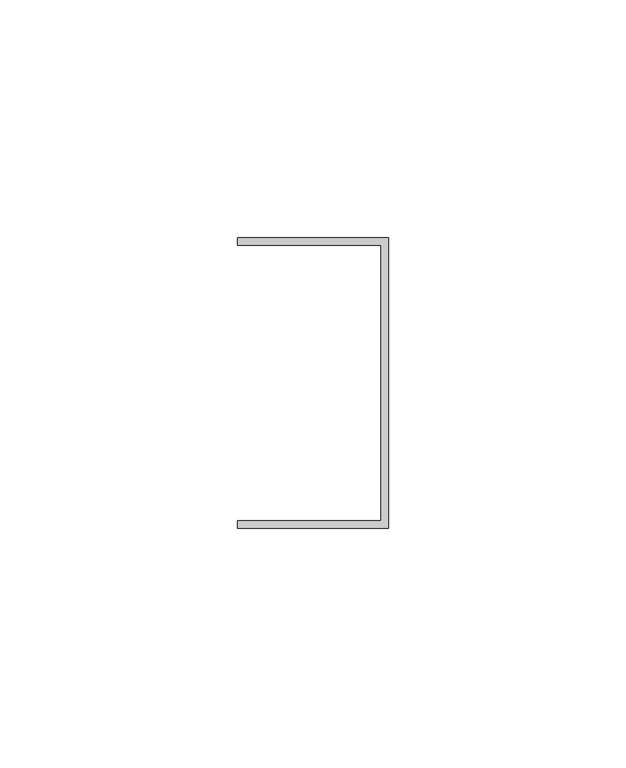
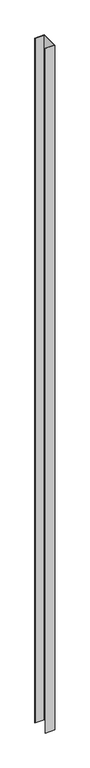
"""IFC4 building model written with IfcOpenShell, lengths in millimetres: proxy geometry, Generic Models 7:Generic Models 1:3:Generic Models 1:3 : Generic Models 7:Generic Models 1:305549:3:Generic Models 1:3:Generic Models 1:3 : Generic Models 7:Generic Models 1:305549:3 : Generic Models 7:Generic Models 1:3:Generic Models 1:3 : Generic Models 7:Generic Models 1:305549:301244:11 : Generic Models 7:Generic Models 1:3:Generic Models 1:3 : Generic Models 7:Generic Models 1:305549:3:Generic Models 1:3:Generic Models 1:3 : Generic Models 7:Generic Models 1:305549:3 : Generic Models 7:Generic Models 1:3:Generic Models 1:3 : Generic Models 7:Generic Models 1:305549:301244:308848."""

from ifc_helpers import new_model, si_unit, frame, origin, place, context, project, spatial, polyline, outline, extrude, source, transform, mapped, element, save


def generic_models_2c4264b5(model_context):
    return source(origin(), model_context, "Body", "SweptSolid", [
        extrude(outline(polyline([(579320.411724, -579015.772634), (579320.411724, -579076.8913841), (579288.661724, -579076.8913841), (579288.661724, -579075.3038841), (579318.824224, -579075.3038841), (579318.824224, -579017.360134), (579288.661724, -579017.360134), (579288.661724, -579015.772634), (579320.411724, -579015.772634)])), frame((0.0, 0.0, 3721.1), z_axis=(0.0, 0.0, 1.0), x_axis=(1.0, 0.0, 0.0)), (0.0, 0.0, 1.0), 2430.9324376),
    ])


if __name__ == "__main__":
    model = new_model("IFC4")
    model_context = context("Model", 3, world=origin())
    ifc_project = project(units=[si_unit("LENGTHUNIT", "METRE", prefix="MILLI")], contexts=[model_context])
    site = spatial("IfcSite", under=ifc_project)
    building = spatial("IfcBuilding", under=site)
    placement = place(None, origin())
    generic_models_shape = generic_models_2c4264b5(model_context)
    element("IfcBuildingElementProxy", 1, Name="Generic Models 7:Generic Models 1:3:Generic Models 1:3 : Generic Models 7:Generic Models 1:305549:3:Generic Models 1:3:Generic Models 1:3 : Generic Models 7:Generic Models 1:305549:3 : Generic Models 7:Generic Models 1:3:Generic Models 1:3 : Generic Models 7:Generic Models 1:305549:301244:11 : Generic Models 7:Generic Models 1:3:Generic Models 1:3 : Generic Models 7:Generic Models 1:305549:3:Generic Models 1:3:Generic Models 1:3 : Generic Models 7:Generic Models 1:305549:3 : Generic Models 7:Generic Models 1:3:Generic Models 1:3 : Generic Models 7:Generic Models 1:305549:301244:308848", ObjectType="Generic Models 7:Generic Models 1:3:Generic Models 1:3 : Generic Models 7:Generic Models 1:305549:3:Generic Models 1:3:Generic Models 1:3 : Generic Models 7:Generic Models 1:305549:3 : Generic Models 7:Generic Models 1:3:Generic Models 1:3 : Generic Models 7:Generic Models 1:305549:301244:11 : Generic Models 7:Generic Models 1:3:Generic Models 1:3 : Generic Models 7:Generic Models 1:305549:3:Generic Models 1:3:Generic Models 1:3 : Generic Models 7:Generic Models 1:305549:3 : Generic Models 7:Generic Models 1:3:Generic Models 1:3 : Generic Models 7:Generic Models 1:305549:301244:308848", at=placement, inside=building, context=model_context, shape_type="MappedRepresentation", body=[
        mapped(generic_models_shape, transform((0.0, 0.0, 0.0), x_axis=(1.0, 0.0, 0.0), y_axis=(0.0, 1.0, 0.0), z_axis=(0.0, 0.0, 1.0))),
    ])
    save(model, "model.ifc")

# Revit data of these elements
# Type "Generic Models 7:Generic Models 1:3:Generic Models 1:3 : Generic Models 7:Generic Models 1:305549:3:Generic Models 1:3:Generic Models 1:3 : Generic Models 7:Generic Models 1:305549:3 : Generic Models 7:Generic Models 1:3:Generic Models 1:3 : Generic Models 7:Generic Models 1:305549:301244:11 : Generic Models 7:Generic Models 1:3:Generic Models 1:3 : Generic Models 7:Generic Models 1:305549:3:Generic Models 1:3:Generic Models 1:3 : Generic Models 7:Generic Models 1:305549:3 : Generic Models 7:Generic Models 1:3:Generic Models 1:3 : Generic Models 7:Generic Models 1:305549:301244:308848"
#   NameOverride = "Generic Models 7:Generic Models 1:3:Generic Models 1:3 : Generic Models 7:Generic Models 1:305549:3:Generic Models 1:3:Generic Models 1:3 : Generic Models 7:Generic Models 1:305549:3 : Generic Models 7:Generic Models 1:3:Generic Models 1:3 : Generic Models 7:Generic Models 1:305549:301244:308848"
#   ObjectTypeOverride = "Generic Models 1:3:Generic Models 1:3 : Generic Models 7:Generic Models 1:305549:3 : Generic Models 7:Generic Models 1:3:Generic Models 1:3 : Generic Models 7:Generic Models 1:305549:301244"
#   Reference = "Generic Models 1"
#   Tag = "308848"
# Element 1 (IfcBuildingElementProxy, "Generic Models 7:Generic Models 1:3:Generic Models 1:3 : Generic Models 7:Generic Models 1:305549:3:Generic Models 1:3:Generic Models 1:3 : Generic Models 7:Generic Models 1:305549:3 : Generic Models 7:Generic Models 1:3:Generic Models 1:3 : Generic Models 7:Generic Models 1:305549:301244:11 : Generic Models 7:Generic Models 1:3:Generic Models 1:3 : Generic Models 7:Generic Models 1:305549:3:Generic Models 1:3:Generic Models 1:3 : Generic Models 7:Generic Models 1:305549:3 : Generic Models 7:Generic Models 1:3:Generic Models 1:3 : Generic Models 7:Generic Models 1:305549:301244:308848")
#   Materials on its faces: "GALVANIZED U-CHANNEL (250T125-33)"
# Materials
#   "GALVANIZED U-CHANNEL (250T125-33)": class "Unassigned", colour RGB 202 201 200, transparency 0, Keynote = "M05451300.02", Cost = 0
